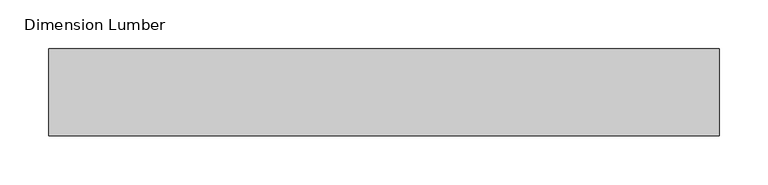
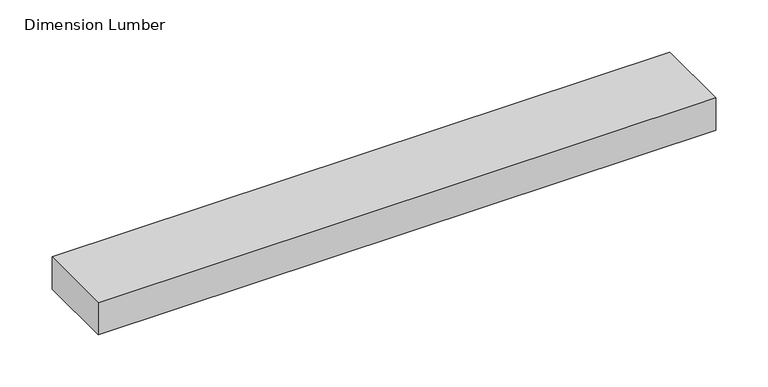
"""IFC4 building model written with IfcOpenShell, lengths in millimetres: beam geometry, Dimension Lumber : Opening Plate 2*4 Exterior."""

from ifc_helpers import new_model, si_unit, frame, origin, place, context, project, spatial, polyline, outline, extrude, source, transform, mapped, element, save


def dimension_lumber_05c0664a(model_context):
    return source(origin(), model_context, "Body", "SweptSolid", [
        extrude(outline(polyline([(333.375, -44.45), (-352.4249994, -44.45), (-352.4249994, 44.45), (333.375, 44.45), (333.375, -44.45)])), frame((0.0, 0.0, -19.05), z_axis=(0.0, 0.0, 1.0), x_axis=(1.0, 0.0, 0.0)), (0.0, 0.0, 1.0), 38.1),
    ])


if __name__ == "__main__":
    model = new_model("IFC4")
    model_context = context("Model", 3, world=origin())
    ifc_project = project(units=[si_unit("LENGTHUNIT", "METRE", prefix="MILLI")], contexts=[model_context])
    site = spatial("IfcSite", under=ifc_project)
    building = spatial("IfcBuilding", under=site)
    placement = place(None, origin())
    dimension_lumber_shape = dimension_lumber_05c0664a(model_context)
    element("IfcBeam", 1, ObjectType="Dimension Lumber : Opening Plate 2*4 Exterior", at=placement, inside=building, context=model_context, shape_type="MappedRepresentation", body=[
        mapped(dimension_lumber_shape, transform((0.0, 0.0, 0.0), x_axis=(1.0, 0.0, 0.0), y_axis=(0.0, 1.0, 0.0), z_axis=(0.0, 0.0, 1.0))),
    ])
    save(model, "model.ifc")

# Revit data of these elements
# Type "Dimension Lumber : Opening Plate 2*4 Exterior"
#   Assembly Code = "B10"
#   A = 0.0364583 SF
#   Length [instance default] = 5' - 0"
#   b = 0' - 3 1/2"
#   d = 0' - 1 1/2"
#   Structural Material [instance default] = Softwood, Lumber
# Element 1 (IfcBeam, "Dimension Lumber : Opening Plate 2*4 Exterior")
#   Structural Material = Douglas Fir #2
#   Materials on its faces: "Douglas Fir #2"
# Materials
#   "Softwood, Lumber": class "Wood", colour RGB 223 192 134, transparency 0, Description = "Pinus Echinata", Cost = 0
#   "Douglas Fir #2": class "Wood", colour RGB 223 192 134, transparency 0, Description = "Pinus Echinata", Cost = 0
